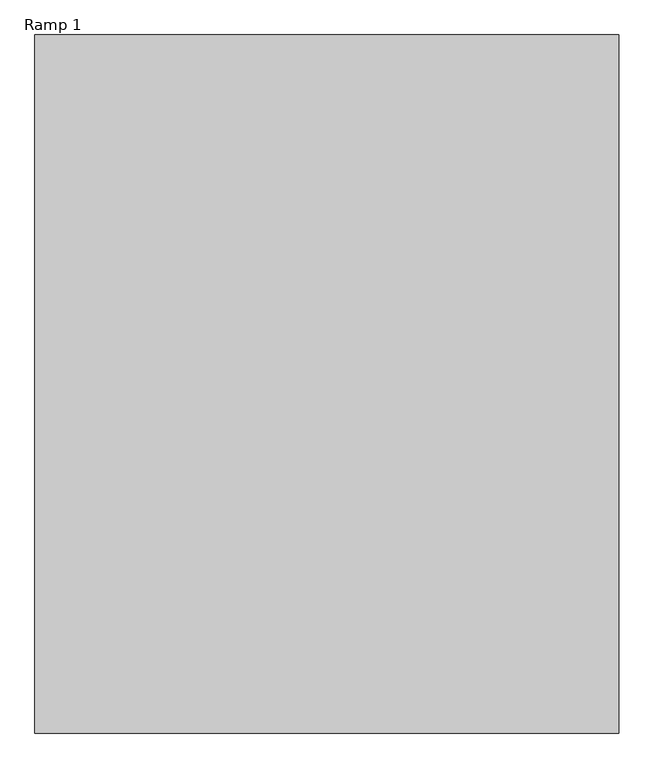
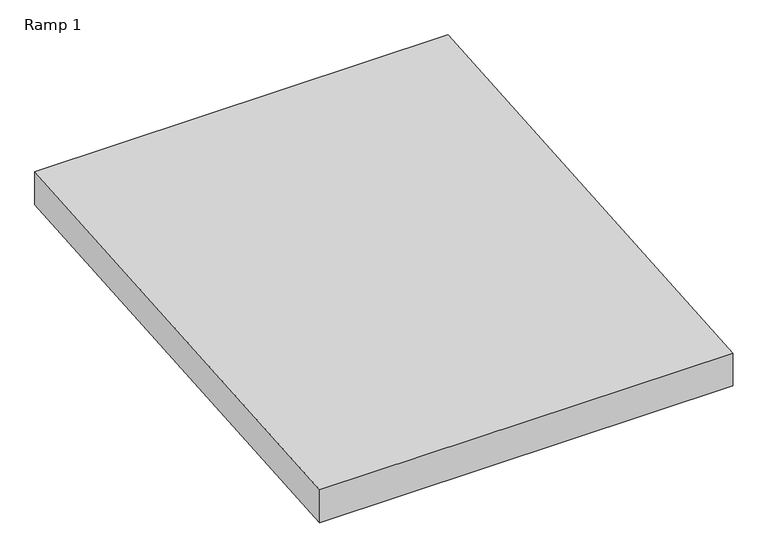
"""IFC4 building model written with IfcOpenShell, lengths in millimetres: ramp geometry, Ramp 1."""

import ifcopenshell
import ifcopenshell.guid

model = None  # the IFC model being written
_history = None  # IfcOwnerHistory: only IFC2X3 demands one
_inside = {}  # id of a spatial element -> (the spatial element, [elements in it])
_under = {}  # id of a project, library or spatial element -> (it, [spatial elements below it])
_declared = {}  # id of a project -> (the project, [libraries it declares])
_typed = {}  # id of a type object -> (the type object, [elements of that type])
_made_of = {}  # id of a material, layer set ... -> (it, [elements and type objects made of it])


def new_model(schema):
    """Start an empty IFC model of exactly this schema.

    Asked for "IFC4X3", IfcOpenShell would pick the latest addendum, in which some entities
    have other attributes; the version numbers below select the first issue.
    IFC2X3 requires an IfcOwnerHistory on every rooted entity: one is made here for all.
    """
    global model, _history
    if schema == "IFC4X3":
        model = ifcopenshell.file(schema_version=(4, 3, 0, 0))
    else:
        model = ifcopenshell.file(schema=schema)
    _inside.clear()
    _under.clear()
    _declared.clear()
    _typed.clear()
    _made_of.clear()
    _history = None
    if model.schema == "IFC2X3":
        org = make("IfcOrganization", Name="unknown")
        user = make(
            "IfcPersonAndOrganization",
            ThePerson=make("IfcPerson", FamilyName="unknown"),
            TheOrganization=org,
        )
        app = make(
            "IfcApplication",
            ApplicationDeveloper=org,
            Version="unknown",
            ApplicationFullName="unknown",
            ApplicationIdentifier="unknown",
        )
        _history = make(
            "IfcOwnerHistory",
            OwningUser=user,
            OwningApplication=app,
            ChangeAction="ADDED",
            CreationDate=0,
        )
    return model


def make(cls, **values):
    """One entity of the class cls with the attributes given. An attribute that is None is left unset."""
    return model.create_entity(
        cls, **{name: value for name, value in values.items() if value is not None}
    )


def rooted(cls, **values):
    """An entity with a GlobalId (a new one), such as an element, a storey or a relation."""
    return make(cls, GlobalId=ifcopenshell.guid.new(), OwnerHistory=_history, **values)


def si_unit(unit_type, name, prefix=None):
    """IfcSIUnit, for example si_unit("LENGTHUNIT", "METRE", prefix="MILLI")."""
    return make("IfcSIUnit", UnitType=unit_type, Prefix=prefix, Name=name)


def assignment(units):
    """IfcUnitAssignment: the units of a project."""
    return None if units is None else make("IfcUnitAssignment", Units=units)


def point(xyz):
    """IfcCartesianPoint."""
    return None if xyz is None else make("IfcCartesianPoint", Coordinates=xyz)


def direction(xyz):
    """IfcDirection."""
    return None if xyz is None else make("IfcDirection", DirectionRatios=xyz)


def frame(location, z_axis=None, x_axis=None):
    """IfcAxis2Placement3D, a coordinate frame: its origin and axes. An axis left out is left unset."""
    return make(
        "IfcAxis2Placement3D",
        Location=point(location),
        Axis=direction(z_axis),
        RefDirection=direction(x_axis),
    )


def origin():
    """The frame at (0, 0, 0) with its axes left unset."""
    return frame((0.0, 0.0, 0.0))


def place(relative_to, where):
    """IfcLocalPlacement: puts the frame where relative to a parent placement (None: the world)."""
    return make(
        "IfcLocalPlacement", PlacementRelTo=relative_to, RelativePlacement=where
    )


def context(
    kind, dimensions, precision=None, world=None, true_north=None, identifier=None
):
    """IfcGeometricRepresentationContext, for example the 3D "Model" context."""
    return make(
        "IfcGeometricRepresentationContext",
        ContextIdentifier=identifier,
        ContextType=kind,
        CoordinateSpaceDimension=dimensions,
        Precision=precision,
        WorldCoordinateSystem=world,
        TrueNorth=true_north,
    )


def project(units=None, contexts=None):
    """IfcProject with its units and contexts."""
    return rooted(
        "IfcProject",
        Name="project",
        RepresentationContexts=contexts,
        UnitsInContext=assignment(units),
    )


def spatial(cls, under=None, at=None, **own):
    """A site, building, storey or space (cls), placed at a placement, below another one or the project."""
    s = rooted(cls, ObjectPlacement=at, **own)
    if under is not None:
        _under.setdefault(under.id(), (under, []))[1].append(s)
    return s


def polyline(points):
    """IfcPolyline through the points."""
    return make("IfcPolyline", Points=[point(p) for p in points])


def outline(outer, holes=None, kind="AREA"):
    """IfcArbitraryClosedProfileDef: a profile drawn as a closed curve; with holes, ...WithVoids."""
    if holes is None:
        return make("IfcArbitraryClosedProfileDef", ProfileType=kind, OuterCurve=outer)
    return make(
        "IfcArbitraryProfileDefWithVoids",
        ProfileType=kind,
        OuterCurve=outer,
        InnerCurves=holes,
    )


def extrude(swept, where, along, depth):
    """IfcExtrudedAreaSolid: the profile swept, set in the frame where, extruded along a direction by depth."""
    return make(
        "IfcExtrudedAreaSolid",
        SweptArea=swept,
        Position=where,
        ExtrudedDirection=direction(along),
        Depth=depth,
    )


def shape(context_of_items, identifier, shape_type, items):
    """IfcShapeRepresentation: the items that make up one representation, for example the "Body"."""
    return make(
        "IfcShapeRepresentation",
        ContextOfItems=context_of_items,
        RepresentationIdentifier=identifier,
        RepresentationType=shape_type,
        Items=items,
    )


def source(mapping_origin, context_of_items, identifier, shape_type, items):
    """IfcRepresentationMap: a shape defined once, which mapped items show again and again."""
    return make(
        "IfcRepresentationMap",
        MappingOrigin=mapping_origin,
        MappedRepresentation=shape(context_of_items, identifier, shape_type, items),
    )


def transform(
    local_origin,
    x_axis=None,
    y_axis=None,
    z_axis=None,
    scale=None,
    scale2=None,
    scale3=None,
    uniform=True,
):
    """IfcCartesianTransformationOperator3D, or its non-uniform kind. x_axis, y_axis, z_axis: its Axis1, 2, 3."""
    if uniform:
        return make(
            "IfcCartesianTransformationOperator3D",
            Axis1=direction(x_axis),
            Axis2=direction(y_axis),
            LocalOrigin=point(local_origin),
            Scale=scale,
            Axis3=direction(z_axis),
        )
    return make(
        "IfcCartesianTransformationOperator3DnonUniform",
        Axis1=direction(x_axis),
        Axis2=direction(y_axis),
        LocalOrigin=point(local_origin),
        Scale=scale,
        Axis3=direction(z_axis),
        Scale2=scale2,
        Scale3=scale3,
    )


def mapped(mapping_source, mapping_target):
    """IfcMappedItem: shows the shape of a source again, moved by a transform."""
    return make(
        "IfcMappedItem", MappingSource=mapping_source, MappingTarget=mapping_target
    )


def made_of(thing, what):
    """Note that an element or type object is made of a material, layer set ...; save() writes the relation."""
    if what is not None:
        _made_of.setdefault(what.id(), (what, []))[1].append(thing)
    return thing


def element(
    cls,
    number,
    at=None,
    inside=None,
    cuts=None,
    type_object=None,
    material=None,
    context=None,
    identifier="Body",
    shape_type=None,
    held_by="IfcProductDefinitionShape",
    body=None,
    shapes=None,
    **own,
):
    """One element of the class cls, such as IfcWall. Its Tag is "e" and its number.

    at: its placement. inside: the storey or other place that contains it. cuts: it is an
    opening in that element (IfcRelVoidsElement). A single representation is given by context,
    identifier, shape_type and body (its items); several are given by shapes. held_by: the class
    of the entity that holds the representations. save() writes the other relations.
    """
    e = rooted(cls, Tag="e%d" % number, ObjectPlacement=at, **own)
    if body is not None:
        shapes = [shape(context, identifier, shape_type, body)]
    if shapes is not None:
        e.Representation = make(held_by, Representations=shapes)
    if inside is not None:
        _inside.setdefault(inside.id(), (inside, []))[1].append(e)
    if cuts is not None:
        rooted(
            "IfcRelVoidsElement", RelatingBuildingElement=cuts, RelatedOpeningElement=e
        )
    if type_object is not None:
        _typed.setdefault(type_object.id(), (type_object, []))[1].append(e)
    return made_of(e, material)


def aggregate(whole, parts):
    """IfcRelAggregates: a whole, such as a stair, and the parts it consists of."""
    return rooted("IfcRelAggregates", RelatingObject=whole, RelatedObjects=parts)


def save(model, path):
    """Write the relations noted so far, then the file.

    IfcRelAggregates (storeys below a building ...), IfcRelContainedInSpatialStructure (elements
    in a storey), IfcRelDefinesByType, IfcRelAssociatesMaterial and IfcRelDeclares: one each for
    every whole, place, type object, material and project.
    """
    for whole, parts in _under.values():
        aggregate(whole, parts)
    for where, things in _inside.values():
        rooted(
            "IfcRelContainedInSpatialStructure",
            RelatedElements=things,
            RelatingStructure=where,
        )
    for kind, things in _typed.values():
        rooted("IfcRelDefinesByType", RelatedObjects=things, RelatingType=kind)
    for what, things in _made_of.values():
        rooted("IfcRelAssociatesMaterial", RelatedObjects=things, RelatingMaterial=what)
    for by, libraries in _declared.values():
        rooted("IfcRelDeclares", RelatingContext=by, RelatedDefinitions=libraries)
    model.write(path)


def ramp_1_66d68c1d(model_context):
    return source(origin(), model_context, "Body", "SweptSolid", [
        extrude(outline(polyline([(-178.9025016, 40.0), (1960.7723822, 200.0), (1960.7723822, 49.5812066), (-178.9025016, -110.4187934), (-178.9025016, 40.0)])), frame((5764.7203549, 0.0, 0.0), z_axis=(1.0, 0.0, 0.0), x_axis=(0.0, 1.0, 0.0)), (0.0, 0.0, 1.0), 1790.0),
    ])


if __name__ == "__main__":
    model = new_model("IFC4")
    model_context = context("Model", 3, world=origin())
    ifc_project = project(units=[si_unit("LENGTHUNIT", "METRE", prefix="MILLI")], contexts=[model_context])
    site = spatial("IfcSite", under=ifc_project)
    building = spatial("IfcBuilding", under=site)
    placement = place(None, origin())
    ramp_1_shape = ramp_1_66d68c1d(model_context)
    element("IfcRamp", 1, ObjectType="Ramp 1", at=placement, inside=building, context=model_context, shape_type="MappedRepresentation", body=[
        mapped(ramp_1_shape, transform((0.0, 0.0, 0.0), x_axis=(1.0, 0.0, 0.0), y_axis=(0.0, 1.0, 0.0), z_axis=(0.0, 0.0, 1.0))),
    ])
    save(model, "model.ifc")
